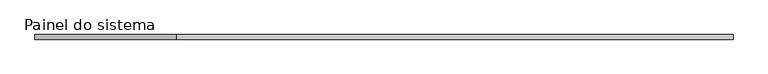
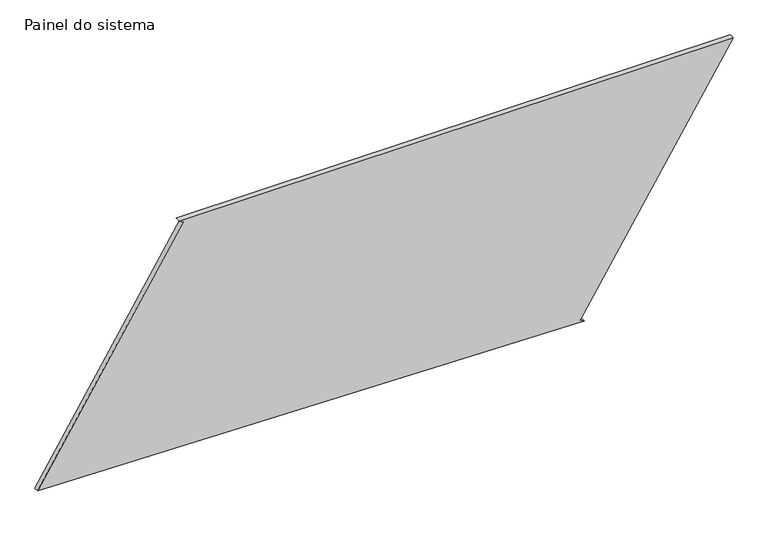
"""IFC4 building model written with IfcOpenShell, lengths in millimetres: plate geometry, Painel do sistema : Envidraçado."""

from ifc_helpers import new_model, si_unit, frame, origin, place, context, project, spatial, polyline, outline, extrude, source, transform, mapped, element, save


def painel_do_sistema_9c9a052f(model_context):
    return source(origin(), model_context, "Body", "SweptSolid", [
        extrude(outline(polyline([(0.0, 1077.9551025), (13.2016257, 1056.725004), (1342.2788796, 1883.1922251), (1342.2788796, -1116.8279447), (1329.0772539, -1095.5978463), (62.5130787, -1883.1922251), (0.0, 1077.9551025)])), frame((0.0, 24.5, 0.0), z_axis=(0.0, 1.0, 0.0), x_axis=(0.0, 0.0, 1.0)), (0.0, 0.0, 1.0), 25.0),
    ])


if __name__ == "__main__":
    model = new_model("IFC4")
    model_context = context("Model", 3, world=origin())
    ifc_project = project(units=[si_unit("LENGTHUNIT", "METRE", prefix="MILLI")], contexts=[model_context])
    site = spatial("IfcSite", under=ifc_project)
    building = spatial("IfcBuilding", under=site)
    placement = place(None, origin())
    painel_do_sistema_shape = painel_do_sistema_9c9a052f(model_context)
    element("IfcPlate", 1, ObjectType="Painel do sistema : Envidraçado", at=placement, inside=building, context=model_context, shape_type="MappedRepresentation", body=[
        mapped(painel_do_sistema_shape, transform((0.0, 0.0, 0.0), x_axis=(1.0, 0.0, 0.0), y_axis=(0.0, 1.0, 0.0), z_axis=(0.0, 0.0, 1.0))),
    ])
    save(model, "model.ifc")

# Revit data of these elements
# Type "Painel do sistema : Envidraçado"
#   Construction Type Id = "GSP4R"
#   Analytic Construction = "Vidraça única Pilkington 1/8 pol"
#   Visual Light Transmittance = 0.9
#   Solar Heat Gain Coefficient = 0.86
#   Heat Transfer Coefficient (U) = 6.7069 W/(m²·K)
# Element 1 (IfcPlate, "Painel do sistema : Envidraçado")
#   Materials on its faces: "Vidro"
# Materials
#   "Vidro": class "Vidro", colour RGB 0 128 192, transparency 0.9, Description = "Vidro de sílica", Cost = 0
